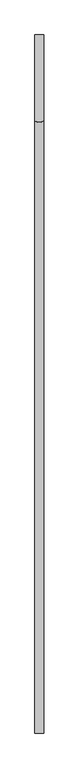
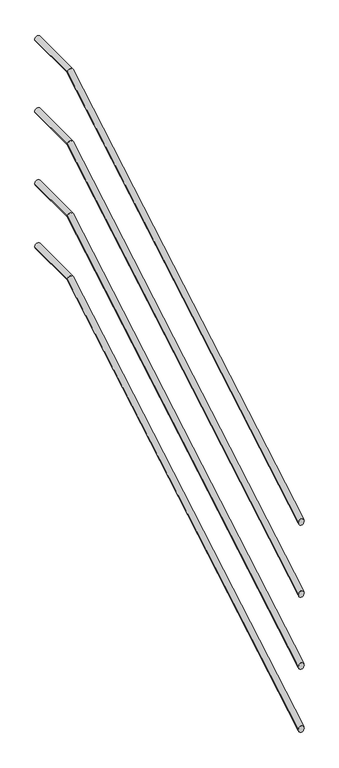
"""IFC4 building model written with IfcOpenShell, lengths in millimetres: railing geometry."""

import ifcopenshell
import ifcopenshell.guid

model = None  # the IFC model being written
_history = None  # IfcOwnerHistory: only IFC2X3 demands one
_inside = {}  # id of a spatial element -> (the spatial element, [elements in it])
_under = {}  # id of a project, library or spatial element -> (it, [spatial elements below it])
_declared = {}  # id of a project -> (the project, [libraries it declares])
_typed = {}  # id of a type object -> (the type object, [elements of that type])
_made_of = {}  # id of a material, layer set ... -> (it, [elements and type objects made of it])


def new_model(schema):
    """Start an empty IFC model of exactly this schema.

    Asked for "IFC4X3", IfcOpenShell would pick the latest addendum, in which some entities
    have other attributes; the version numbers below select the first issue.
    IFC2X3 requires an IfcOwnerHistory on every rooted entity: one is made here for all.
    """
    global model, _history
    if schema == "IFC4X3":
        model = ifcopenshell.file(schema_version=(4, 3, 0, 0))
    else:
        model = ifcopenshell.file(schema=schema)
    _inside.clear()
    _under.clear()
    _declared.clear()
    _typed.clear()
    _made_of.clear()
    _history = None
    if model.schema == "IFC2X3":
        org = make("IfcOrganization", Name="unknown")
        user = make(
            "IfcPersonAndOrganization",
            ThePerson=make("IfcPerson", FamilyName="unknown"),
            TheOrganization=org,
        )
        app = make(
            "IfcApplication",
            ApplicationDeveloper=org,
            Version="unknown",
            ApplicationFullName="unknown",
            ApplicationIdentifier="unknown",
        )
        _history = make(
            "IfcOwnerHistory",
            OwningUser=user,
            OwningApplication=app,
            ChangeAction="ADDED",
            CreationDate=0,
        )
    return model


def make(cls, **values):
    """One entity of the class cls with the attributes given. An attribute that is None is left unset."""
    return model.create_entity(
        cls, **{name: value for name, value in values.items() if value is not None}
    )


def rooted(cls, **values):
    """An entity with a GlobalId (a new one), such as an element, a storey or a relation."""
    return make(cls, GlobalId=ifcopenshell.guid.new(), OwnerHistory=_history, **values)


def si_unit(unit_type, name, prefix=None):
    """IfcSIUnit, for example si_unit("LENGTHUNIT", "METRE", prefix="MILLI")."""
    return make("IfcSIUnit", UnitType=unit_type, Prefix=prefix, Name=name)


def assignment(units):
    """IfcUnitAssignment: the units of a project."""
    return None if units is None else make("IfcUnitAssignment", Units=units)


def point(xyz):
    """IfcCartesianPoint."""
    return None if xyz is None else make("IfcCartesianPoint", Coordinates=xyz)


def direction(xyz):
    """IfcDirection."""
    return None if xyz is None else make("IfcDirection", DirectionRatios=xyz)


def frame(location, z_axis=None, x_axis=None):
    """IfcAxis2Placement3D, a coordinate frame: its origin and axes. An axis left out is left unset."""
    return make(
        "IfcAxis2Placement3D",
        Location=point(location),
        Axis=direction(z_axis),
        RefDirection=direction(x_axis),
    )


def origin():
    """The frame at (0, 0, 0) with its axes left unset."""
    return frame((0.0, 0.0, 0.0))


def place(relative_to, where):
    """IfcLocalPlacement: puts the frame where relative to a parent placement (None: the world)."""
    return make(
        "IfcLocalPlacement", PlacementRelTo=relative_to, RelativePlacement=where
    )


def context(
    kind, dimensions, precision=None, world=None, true_north=None, identifier=None
):
    """IfcGeometricRepresentationContext, for example the 3D "Model" context."""
    return make(
        "IfcGeometricRepresentationContext",
        ContextIdentifier=identifier,
        ContextType=kind,
        CoordinateSpaceDimension=dimensions,
        Precision=precision,
        WorldCoordinateSystem=world,
        TrueNorth=true_north,
    )


def project(units=None, contexts=None):
    """IfcProject with its units and contexts."""
    return rooted(
        "IfcProject",
        Name="project",
        RepresentationContexts=contexts,
        UnitsInContext=assignment(units),
    )


def spatial(cls, under=None, at=None, **own):
    """A site, building, storey or space (cls), placed at a placement, below another one or the project."""
    s = rooted(cls, ObjectPlacement=at, **own)
    if under is not None:
        _under.setdefault(under.id(), (under, []))[1].append(s)
    return s


def circle_curve(where, radius):
    """IfcCircle in the frame where."""
    return make("IfcCircle", Position=where, Radius=radius)


def ellipse_curve(where, semi_axis1, semi_axis2):
    """IfcEllipse in the frame where."""
    return make(
        "IfcEllipse", Position=where, SemiAxis1=semi_axis1, SemiAxis2=semi_axis2
    )


def shape(context_of_items, identifier, shape_type, items):
    """IfcShapeRepresentation: the items that make up one representation, for example the "Body"."""
    return make(
        "IfcShapeRepresentation",
        ContextOfItems=context_of_items,
        RepresentationIdentifier=identifier,
        RepresentationType=shape_type,
        Items=items,
    )


def source(mapping_origin, context_of_items, identifier, shape_type, items):
    """IfcRepresentationMap: a shape defined once, which mapped items show again and again."""
    return make(
        "IfcRepresentationMap",
        MappingOrigin=mapping_origin,
        MappedRepresentation=shape(context_of_items, identifier, shape_type, items),
    )


def transform(
    local_origin,
    x_axis=None,
    y_axis=None,
    z_axis=None,
    scale=None,
    scale2=None,
    scale3=None,
    uniform=True,
):
    """IfcCartesianTransformationOperator3D, or its non-uniform kind. x_axis, y_axis, z_axis: its Axis1, 2, 3."""
    if uniform:
        return make(
            "IfcCartesianTransformationOperator3D",
            Axis1=direction(x_axis),
            Axis2=direction(y_axis),
            LocalOrigin=point(local_origin),
            Scale=scale,
            Axis3=direction(z_axis),
        )
    return make(
        "IfcCartesianTransformationOperator3DnonUniform",
        Axis1=direction(x_axis),
        Axis2=direction(y_axis),
        LocalOrigin=point(local_origin),
        Scale=scale,
        Axis3=direction(z_axis),
        Scale2=scale2,
        Scale3=scale3,
    )


def mapped(mapping_source, mapping_target):
    """IfcMappedItem: shows the shape of a source again, moved by a transform."""
    return make(
        "IfcMappedItem", MappingSource=mapping_source, MappingTarget=mapping_target
    )


def made_of(thing, what):
    """Note that an element or type object is made of a material, layer set ...; save() writes the relation."""
    if what is not None:
        _made_of.setdefault(what.id(), (what, []))[1].append(thing)
    return thing


def element(
    cls,
    number,
    at=None,
    inside=None,
    cuts=None,
    type_object=None,
    material=None,
    context=None,
    identifier="Body",
    shape_type=None,
    held_by="IfcProductDefinitionShape",
    body=None,
    shapes=None,
    **own,
):
    """One element of the class cls, such as IfcWall. Its Tag is "e" and its number.

    at: its placement. inside: the storey or other place that contains it. cuts: it is an
    opening in that element (IfcRelVoidsElement). A single representation is given by context,
    identifier, shape_type and body (its items); several are given by shapes. held_by: the class
    of the entity that holds the representations. save() writes the other relations.
    """
    e = rooted(cls, Tag="e%d" % number, ObjectPlacement=at, **own)
    if body is not None:
        shapes = [shape(context, identifier, shape_type, body)]
    if shapes is not None:
        e.Representation = make(held_by, Representations=shapes)
    if inside is not None:
        _inside.setdefault(inside.id(), (inside, []))[1].append(e)
    if cuts is not None:
        rooted(
            "IfcRelVoidsElement", RelatingBuildingElement=cuts, RelatedOpeningElement=e
        )
    if type_object is not None:
        _typed.setdefault(type_object.id(), (type_object, []))[1].append(e)
    return made_of(e, material)


def aggregate(whole, parts):
    """IfcRelAggregates: a whole, such as a stair, and the parts it consists of."""
    return rooted("IfcRelAggregates", RelatingObject=whole, RelatedObjects=parts)


def save(model, path):
    """Write the relations noted so far, then the file.

    IfcRelAggregates (storeys below a building ...), IfcRelContainedInSpatialStructure (elements
    in a storey), IfcRelDefinesByType, IfcRelAssociatesMaterial and IfcRelDeclares: one each for
    every whole, place, type object, material and project.
    """
    for whole, parts in _under.values():
        aggregate(whole, parts)
    for where, things in _inside.values():
        rooted(
            "IfcRelContainedInSpatialStructure",
            RelatedElements=things,
            RelatingStructure=where,
        )
    for kind, things in _typed.values():
        rooted("IfcRelDefinesByType", RelatedObjects=things, RelatingType=kind)
    for what, things in _made_of.values():
        rooted("IfcRelAssociatesMaterial", RelatedObjects=things, RelatingMaterial=what)
    for by, libraries in _declared.values():
        rooted("IfcRelDeclares", RelatingContext=by, RelatedDefinitions=libraries)
    model.write(path)


def plane_surface(at):
    """IfcPlane: the flat surface through the origin of the frame at, square to its z axis."""
    return make("IfcPlane", Position=at)


def cylinder_surface(at, radius):
    """IfcCylindricalSurface: all points at the distance radius from the z axis of the frame at."""
    return make("IfcCylindricalSurface", Position=at, Radius=radius)


def advanced_brep(points, edges, surfaces, faces):
    """IfcAdvancedBrep: a solid bounded by faces that lie on surfaces and meet in shared edges.

    An edge is (start, end): straight between two places in points (the first is 0);
    or (start, end, curve); or (start, end, curve, False) where it runs against its curve.
    A face is (place in surfaces, loops), or (place, loops, False) where it looks against
    its surface's normal. A loop lists edges by number (the first is 1), with a minus sign
    where the edge is run from its end to its start. The first loop is the outer one.
    """
    corners = [point(p) for p in points]
    vertices = [make("IfcVertexPoint", VertexGeometry=c) for c in corners]
    made = []
    for start, end, *more in edges:
        made.append(
            make(
                "IfcEdgeCurve",
                EdgeStart=vertices[start],
                EdgeEnd=vertices[end],
                EdgeGeometry=more[0] if more else make("IfcPolyline", Points=[corners[start], corners[end]]),
                SameSense=more[1] if len(more) > 1 else True,
            )
        )
    hull = []
    for where, loops, *sense in faces:
        bounds = []
        for j, loop in enumerate(loops):
            ring = [make("IfcOrientedEdge", EdgeElement=made[abs(k) - 1], Orientation=k > 0) for k in loop]
            bounds.append(
                make(
                    "IfcFaceOuterBound" if j == 0 else "IfcFaceBound",
                    Bound=make("IfcEdgeLoop", EdgeList=ring),
                    Orientation=True,
                )
            )
        hull.append(make("IfcAdvancedFace", Bounds=bounds, FaceSurface=surfaces[where], SameSense=sense[0] if sense else True))
    return make("IfcAdvancedBrep", Outer=make("IfcClosedShell", CfsFaces=hull))


def railing_f234ddb2(model_context):
    return source(origin(), model_context, "Body", "AdvancedBrep", [
        advanced_brep(
        [(-1890.4, 13399.5208589, 7257.5963084), (-1860.4, 13399.5208589, 7257.5963084), (-1890.4, 15503.576096, 8484.9618634), (-1860.4, 15503.576096, 8484.9618634), (-1890.4, 15799.5208589, 8484.9618634), (-1860.4, 15799.5208589, 8484.9618634)],
        [
            (0, 1, ellipse_curve(frame((-1875.4, 13399.5208589, 7257.5963084), z_axis=(0.0, -1.0, 0.0), x_axis=(0.0, 0.0, -1.0)), 17.365555, 15.0)),
            (1, 0, ellipse_curve(frame((-1875.4, 13399.5208589, 7257.5963084), z_axis=(0.0, -1.0, 0.0), x_axis=(0.0, 0.0, -1.0)), 17.365555, 15.0)),
            (0, 2),
            (2, 3, ellipse_curve(frame((-1875.4, 15503.576096, 8484.9618634), z_axis=(0.0, -0.965344213454049, -0.26097997921446653), x_axis=(0.0, 0.2609799792144656, -0.9653442134540494)), 15.5384989, 15.0)),
            (3, 1),
            (3, 2, ellipse_curve(frame((-1875.4, 15503.576096, 8484.9618634), z_axis=(0.0, -0.965344213454049, -0.26097997921446653), x_axis=(0.0, 0.2609799792144656, -0.9653442134540494)), 15.5384989, 15.0)),
            (4, 5, circle_curve(frame((-1875.4, 15799.5208589, 8484.9618634), z_axis=(0.0, 1.0, 0.0), x_axis=(1.0, 0.0, 0.0)), 15.0)),
            (5, 4, circle_curve(frame((-1875.4, 15799.5208589, 8484.9618634), z_axis=(0.0, 1.0, 0.0), x_axis=(1.0, 0.0, 0.0)), 15.0)),
            (2, 4),
            (5, 3),
        ],
        [
            plane_surface(frame((-1875.4, 13399.5208589, 7274.9618634), z_axis=(0.0, -1.0, 0.0), x_axis=(0.0, 0.0, 1.0))),
            cylinder_surface(frame((-1875.4, 13407.0789243, 7262.0051799), z_axis=(0.0, -0.8637789008984332, -0.5038710255240865), x_axis=(1.0, 0.0, 0.0)), 15.0),
            plane_surface(frame((-1875.4, 15799.5208589, 8499.9618634), z_axis=(0.0, 1.0, 0.0), x_axis=(0.0, 0.0, 1.0))),
            cylinder_surface(frame((-1875.4, 15499.5208589, 8484.9618634), z_axis=(0.0, -1.0, 0.0), x_axis=(1.0, 0.0, 0.0)), 15.0),
        ],
        [
            (0, [[1, 2]]),
            (1, [[-1, 3, 4, 5]]),
            (1, [[-2, -5, 6, -3]]),
            (2, [[7, 8]]),
            (3, [[-4, 9, -8, 10]]),
            (3, [[-6, -10, -7, -9]]),
        ],
    ),
        advanced_brep(
        [(-1890.4, 13399.5208589, 6457.5963084), (-1860.4, 13399.5208589, 6457.5963084), (-1890.4, 15503.576096, 7684.9618634), (-1860.4, 15503.576096, 7684.9618634), (-1890.4, 15799.5208589, 7684.9618634), (-1860.4, 15799.5208589, 7684.9618634)],
        [
            (0, 1, ellipse_curve(frame((-1875.4, 13399.5208589, 6457.5963084), z_axis=(0.0, -1.0, 0.0), x_axis=(0.0, 0.0, -1.0)), 17.365555, 15.0)),
            (1, 0, ellipse_curve(frame((-1875.4, 13399.5208589, 6457.5963084), z_axis=(0.0, -1.0, 0.0), x_axis=(0.0, 0.0, -1.0)), 17.365555, 15.0)),
            (0, 2),
            (2, 3, ellipse_curve(frame((-1875.4, 15503.576096, 7684.9618634), z_axis=(0.0, -0.965344213454049, -0.26097997921446653), x_axis=(0.0, 0.2609799792144656, -0.9653442134540494)), 15.5384989, 15.0)),
            (3, 1),
            (3, 2, ellipse_curve(frame((-1875.4, 15503.576096, 7684.9618634), z_axis=(0.0, -0.965344213454049, -0.26097997921446653), x_axis=(0.0, 0.2609799792144656, -0.9653442134540494)), 15.5384989, 15.0)),
            (4, 5, circle_curve(frame((-1875.4, 15799.5208589, 7684.9618634), z_axis=(0.0, 1.0, 0.0), x_axis=(1.0, 0.0, 0.0)), 15.0)),
            (5, 4, circle_curve(frame((-1875.4, 15799.5208589, 7684.9618634), z_axis=(0.0, 1.0, 0.0), x_axis=(1.0, 0.0, 0.0)), 15.0)),
            (2, 4),
            (5, 3),
        ],
        [
            plane_surface(frame((-1875.4, 13399.5208589, 6474.9618634), z_axis=(0.0, -1.0, 0.0), x_axis=(0.0, 0.0, 1.0))),
            cylinder_surface(frame((-1875.4, 13407.0789243, 6462.0051799), z_axis=(0.0, -0.8637789008984332, -0.5038710255240865), x_axis=(1.0, 0.0, 0.0)), 15.0),
            plane_surface(frame((-1875.4, 15799.5208589, 7699.9618634), z_axis=(0.0, 1.0, 0.0), x_axis=(0.0, 0.0, 1.0))),
            cylinder_surface(frame((-1875.4, 15499.5208589, 7684.9618634), z_axis=(0.0, -1.0, 0.0), x_axis=(1.0, 0.0, 0.0)), 15.0),
        ],
        [
            (0, [[1, 2]]),
            (1, [[-1, 3, 4, 5]]),
            (1, [[-2, -5, 6, -3]]),
            (2, [[7, 8]]),
            (3, [[-4, 9, -8, 10]]),
            (3, [[-6, -10, -7, -9]]),
        ],
    ),
        advanced_brep(
        [(-1890.4, 13399.5208589, 6857.5963084), (-1860.4, 13399.5208589, 6857.5963084), (-1890.4, 15503.576096, 8084.9618634), (-1860.4, 15503.576096, 8084.9618634), (-1890.4, 15799.5208589, 8084.9618634), (-1860.4, 15799.5208589, 8084.9618634)],
        [
            (0, 1, ellipse_curve(frame((-1875.4, 13399.5208589, 6857.5963084), z_axis=(0.0, -1.0, 0.0), x_axis=(0.0, 0.0, -1.0)), 17.365555, 15.0)),
            (1, 0, ellipse_curve(frame((-1875.4, 13399.5208589, 6857.5963084), z_axis=(0.0, -1.0, 0.0), x_axis=(0.0, 0.0, -1.0)), 17.365555, 15.0)),
            (0, 2),
            (2, 3, ellipse_curve(frame((-1875.4, 15503.576096, 8084.9618634), z_axis=(0.0, -0.965344213454049, -0.26097997921446653), x_axis=(0.0, 0.2609799792144656, -0.9653442134540494)), 15.5384989, 15.0)),
            (3, 1),
            (3, 2, ellipse_curve(frame((-1875.4, 15503.576096, 8084.9618634), z_axis=(0.0, -0.965344213454049, -0.26097997921446653), x_axis=(0.0, 0.2609799792144656, -0.9653442134540494)), 15.5384989, 15.0)),
            (4, 5, circle_curve(frame((-1875.4, 15799.5208589, 8084.9618634), z_axis=(0.0, 1.0, 0.0), x_axis=(1.0, 0.0, 0.0)), 15.0)),
            (5, 4, circle_curve(frame((-1875.4, 15799.5208589, 8084.9618634), z_axis=(0.0, 1.0, 0.0), x_axis=(1.0, 0.0, 0.0)), 15.0)),
            (2, 4),
            (5, 3),
        ],
        [
            plane_surface(frame((-1875.4, 13399.5208589, 6874.9618634), z_axis=(0.0, -1.0, 0.0), x_axis=(0.0, 0.0, 1.0))),
            cylinder_surface(frame((-1875.4, 13407.0789243, 6862.0051799), z_axis=(0.0, -0.8637789008984332, -0.5038710255240865), x_axis=(1.0, 0.0, 0.0)), 15.0),
            plane_surface(frame((-1875.4, 15799.5208589, 8099.9618634), z_axis=(0.0, 1.0, 0.0), x_axis=(0.0, 0.0, 1.0))),
            cylinder_surface(frame((-1875.4, 15499.5208589, 8084.9618634), z_axis=(0.0, -1.0, 0.0), x_axis=(1.0, 0.0, 0.0)), 15.0),
        ],
        [
            (0, [[1, 2]]),
            (1, [[-1, 3, 4, 5]]),
            (1, [[-2, -5, 6, -3]]),
            (2, [[7, 8]]),
            (3, [[-4, 9, -8, 10]]),
            (3, [[-6, -10, -7, -9]]),
        ],
    ),
        advanced_brep(
        [(-1890.4, 13399.5208589, 6107.5963084), (-1860.4, 13399.5208589, 6107.5963084), (-1890.4, 15503.576096, 7334.9618634), (-1860.4, 15503.576096, 7334.9618634), (-1890.4, 15799.5208589, 7334.9618634), (-1860.4, 15799.5208589, 7334.9618634)],
        [
            (0, 1, ellipse_curve(frame((-1875.4, 13399.5208589, 6107.5963084), z_axis=(0.0, -1.0, 0.0), x_axis=(0.0, 0.0, -1.0)), 17.365555, 15.0)),
            (1, 0, ellipse_curve(frame((-1875.4, 13399.5208589, 6107.5963084), z_axis=(0.0, -1.0, 0.0), x_axis=(0.0, 0.0, -1.0)), 17.365555, 15.0)),
            (0, 2),
            (2, 3, ellipse_curve(frame((-1875.4, 15503.576096, 7334.9618634), z_axis=(0.0, -0.965344213454049, -0.26097997921446653), x_axis=(0.0, 0.2609799792144656, -0.9653442134540494)), 15.5384989, 15.0)),
            (3, 1),
            (3, 2, ellipse_curve(frame((-1875.4, 15503.576096, 7334.9618634), z_axis=(0.0, -0.965344213454049, -0.26097997921446653), x_axis=(0.0, 0.2609799792144656, -0.9653442134540494)), 15.5384989, 15.0)),
            (4, 5, circle_curve(frame((-1875.4, 15799.5208589, 7334.9618634), z_axis=(0.0, 1.0, 0.0), x_axis=(1.0, 0.0, 0.0)), 15.0)),
            (5, 4, circle_curve(frame((-1875.4, 15799.5208589, 7334.9618634), z_axis=(0.0, 1.0, 0.0), x_axis=(1.0, 0.0, 0.0)), 15.0)),
            (2, 4),
            (5, 3),
        ],
        [
            plane_surface(frame((-1875.4, 13399.5208589, 6124.9618634), z_axis=(0.0, -1.0, 0.0), x_axis=(0.0, 0.0, 1.0))),
            cylinder_surface(frame((-1875.4, 13407.0789243, 6112.0051799), z_axis=(0.0, -0.8637789008984332, -0.5038710255240865), x_axis=(1.0, 0.0, 0.0)), 15.0),
            plane_surface(frame((-1875.4, 15799.5208589, 7349.9618634), z_axis=(0.0, 1.0, 0.0), x_axis=(0.0, 0.0, 1.0))),
            cylinder_surface(frame((-1875.4, 15499.5208589, 7334.9618634), z_axis=(0.0, -1.0, 0.0), x_axis=(1.0, 0.0, 0.0)), 15.0),
        ],
        [
            (0, [[1, 2]]),
            (1, [[-1, 3, 4, 5]]),
            (1, [[-2, -5, 6, -3]]),
            (2, [[7, 8]]),
            (3, [[-4, 9, -8, 10]]),
            (3, [[-6, -10, -7, -9]]),
        ],
    ),
    ])


if __name__ == "__main__":
    model = new_model("IFC4")
    model_context = context("Model", 3, world=origin())
    ifc_project = project(units=[si_unit("LENGTHUNIT", "METRE", prefix="MILLI")], contexts=[model_context])
    site = spatial("IfcSite", under=ifc_project)
    building = spatial("IfcBuilding", under=site)
    placement = place(None, origin())
    railing_shape = railing_f234ddb2(model_context)
    element("IfcRailing", 1, at=placement, inside=building, context=model_context, shape_type="MappedRepresentation", body=[
        mapped(railing_shape, transform((0.0, 0.0, 0.0), x_axis=(1.0, 0.0, 0.0), y_axis=(0.0, 1.0, 0.0), z_axis=(0.0, 0.0, 1.0))),
    ])
    save(model, "model.ifc")
